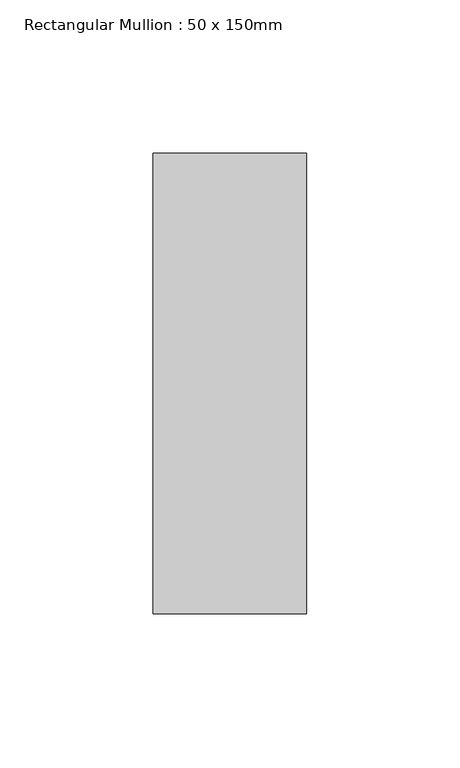
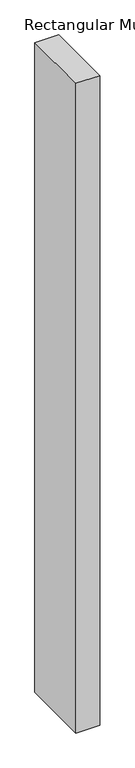
"""IFC4 building model written with IfcOpenShell, lengths in millimetres: member geometry, Rectangular Mullion : 50 x 150mm."""

from ifc_helpers import new_model, si_unit, frame, origin, place, context, project, spatial, polyline, outline, extrude, source, transform, mapped, element, save


def rectangular_mullion_50_x_150mm_a4200a9d(model_context):
    return source(origin(), model_context, "Body", "SweptSolid", [
        extrude(outline(polyline([(25.0, 75.0), (25.0, -75.0), (-25.0, -75.0), (-25.0, 75.0), (25.0, 75.0)])), frame((0.0, 0.0, -1450.1029933), z_axis=(0.0, 0.0, 1.0), x_axis=(1.0, 0.0, 0.0)), (0.0, 0.0, 1.0), 1450.1029933),
    ])


if __name__ == "__main__":
    model = new_model("IFC4")
    model_context = context("Model", 3, world=origin())
    ifc_project = project(units=[si_unit("LENGTHUNIT", "METRE", prefix="MILLI")], contexts=[model_context])
    site = spatial("IfcSite", under=ifc_project)
    building = spatial("IfcBuilding", under=site)
    placement = place(None, origin())
    rectangular_mullion_50_x_150mm_shape = rectangular_mullion_50_x_150mm_a4200a9d(model_context)
    element("IfcMember", 1, ObjectType="Rectangular Mullion : 50 x 150mm", at=placement, inside=building, context=model_context, shape_type="MappedRepresentation", body=[
        mapped(rectangular_mullion_50_x_150mm_shape, transform((0.0, 0.0, 0.0), x_axis=(1.0, 0.0, 0.0), y_axis=(0.0, 1.0, 0.0), z_axis=(0.0, 0.0, 1.0))),
    ])
    save(model, "model.ifc")

# Revit data of these elements
# Type "Rectangular Mullion : 50 x 150mm"
#   Keynote = "H11"
#   built-in parameter 1007304 = 0.492126 (stored number, unit not read)
#   built-in parameter 1007301 = 0.082021 (stored number, unit not read)
#   built-in parameter 1007300 = 0.082021 (stored number, unit not read)
# Element 1 (IfcMember, "Rectangular Mullion : 50 x 150mm")
#   Materials on its faces: "Aluminium"
# Materials
#   "Aluminium": class "Metal", colour RGB 247 247 247, transparency 0, Description = "Aluminium 6061", Cost = 0
